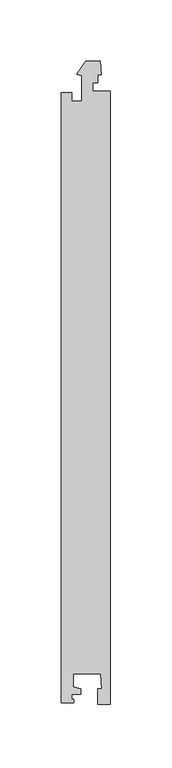
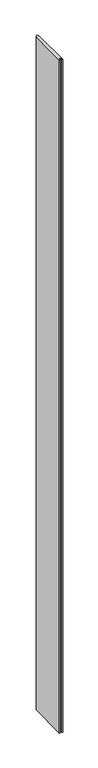
"""IFC4 building model written with IfcOpenShell, lengths in millimetres: proxy geometry, Generic Models 5:Generic Models 5:321804:Generic Models 5:321804 : Generic Models 5:Generic Models 5:321804:32 : Generic Models 5:Generic Models 5:321804:Generic Models 5:321804 : Generic Models 5:Generic Models 5:321804:300761."""

from ifc_helpers import new_model, si_unit, frame, origin, place, context, project, spatial, polyline, outline, extrude, source, transform, mapped, element, save


def generic_models_be12d552(model_context):
    return source(origin(), model_context, "Body", "SweptSolid", [
        extrude(outline(polyline([(667625.2338797, -493410.833465), (667631.7338797, -493412.5751348), (667631.7338797, -493417.0251348), (667624.2338797, -493417.0251348), (667624.2338797, -493420.9751348), (667625.7338797, -493420.9751348), (667625.7338797, -493423.9751348), (667615.7338797, -493423.9751348), (667615.7338797, -492926.4751348), (667624.2338797, -492926.4751348), (667624.2338797, -492933.4251348), (667632.2338797, -492933.4251348), (667632.2338797, -492912.7091094), (667628.3059983, -492911.6566367), (667635.4133634, -492900.9751348), (667647.2715044, -492900.9751348), (667648.2338797, -492911.9751348), (667645.5338797, -492911.9751348), (667645.5338797, -492918.6001348), (667641.2338797, -492918.6001348), (667641.2338797, -492925.2251348), (667655.7338797, -492925.2251348), (667655.7338797, -493425.2251348), (667645.5338797, -493425.2251348), (667645.5338797, -493412.4751348), (667648.779534, -493412.4751348), (667647.72967, -493400.4751348), (667625.2338797, -493400.4751348), (667625.2338797, -493410.833465)])), frame((0.0, 0.0, -5.8417589), z_axis=(0.0, 0.0, 1.0), x_axis=(1.0, 0.0, 0.0)), (0.0, 0.0, 1.0), 8779.7126309),
    ])


if __name__ == "__main__":
    model = new_model("IFC4")
    model_context = context("Model", 3, world=origin())
    ifc_project = project(units=[si_unit("LENGTHUNIT", "METRE", prefix="MILLI")], contexts=[model_context])
    site = spatial("IfcSite", under=ifc_project)
    building = spatial("IfcBuilding", under=site)
    placement = place(None, origin())
    generic_models_shape = generic_models_be12d552(model_context)
    element("IfcBuildingElementProxy", 1, Name="Generic Models 5:Generic Models 5:321804:Generic Models 5:321804 : Generic Models 5:Generic Models 5:321804:32 : Generic Models 5:Generic Models 5:321804:Generic Models 5:321804 : Generic Models 5:Generic Models 5:321804:300761", ObjectType="Generic Models 5:Generic Models 5:321804:Generic Models 5:321804 : Generic Models 5:Generic Models 5:321804:32 : Generic Models 5:Generic Models 5:321804:Generic Models 5:321804 : Generic Models 5:Generic Models 5:321804:300761", at=placement, inside=building, context=model_context, shape_type="MappedRepresentation", body=[
        mapped(generic_models_shape, transform((0.0, 0.0, 0.0), x_axis=(1.0, 0.0, 0.0), y_axis=(0.0, 1.0, 0.0), z_axis=(0.0, 0.0, 1.0))),
    ])
    save(model, "model.ifc")

# Revit data of these elements
# Type "Generic Models 5:Generic Models 5:321804:Generic Models 5:321804 : Generic Models 5:Generic Models 5:321804:32 : Generic Models 5:Generic Models 5:321804:Generic Models 5:321804 : Generic Models 5:Generic Models 5:321804:300761"
#   NameOverride = "Generic Models 5:Generic Models 5:321804:Generic Models 5:321804 : Generic Models 5:Generic Models 5:321804:300761"
#   ObjectTypeOverride = "Generic Models 5:321804 : Generic Models 5:Generic Models 5:321804"
#   Reference = "Generic Models 5"
#   Tag = "300761"
# Element 1 (IfcBuildingElementProxy, "Generic Models 5:Generic Models 5:321804:Generic Models 5:321804 : Generic Models 5:Generic Models 5:321804:32 : Generic Models 5:Generic Models 5:321804:Generic Models 5:321804 : Generic Models 5:Generic Models 5:321804:300761")
#   Materials on its faces: "POLYCARBONATE PANEL - ARCOPLUS 547"
# Materials
#   "POLYCARBONATE PANEL - ARCOPLUS 547": class "Unassigned", colour RGB 202 225 249, transparency 0.45, Cost = 0
